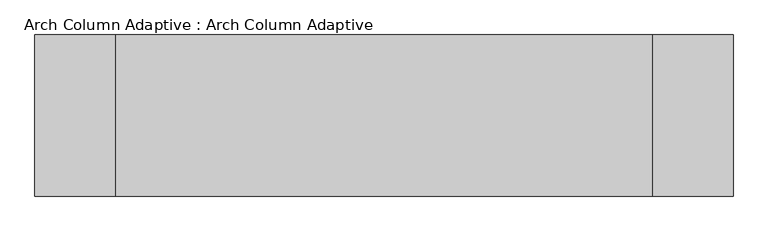
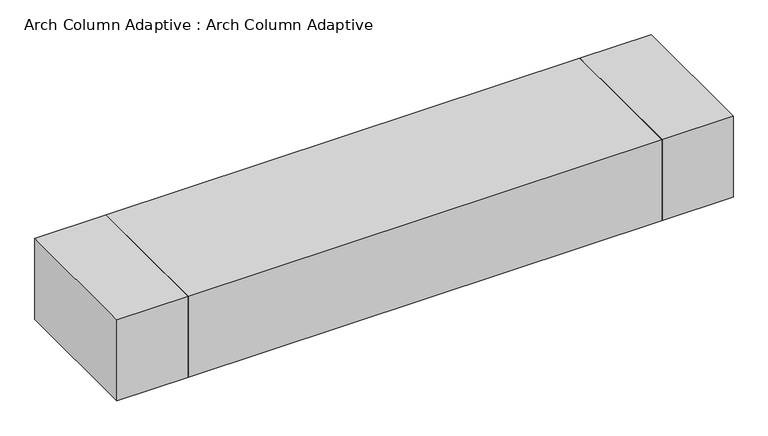
"""IFC4 building model written with IfcOpenShell, lengths in millimetres: proxy geometry, Arch Column Adaptive : Arch Column Adaptive."""

from ifc_helpers import new_model, si_unit, frame, origin, place, context, project, spatial, polyline, outline, extrude, source, transform, mapped, element, save


def arch_column_adaptive_arch_column_adaptive_9be84d25(model_context):
    return source(origin(), model_context, "Body", "SweptSolid", [
        extrude(outline(polyline([(5000.0, -1500.0), (5000.0, 1500.0), (6500.0, 1500.0), (6500.0, -1500.0), (5000.0, -1500.0)])), frame((0.0, 0.0, 79290.0), z_axis=(0.0, 0.0, 1.0), x_axis=(1.0, 0.0, 0.0)), (0.0, 0.0, 1.0), 1800.0),
        extrude(outline(polyline([(-5000.0, 1500.0), (-5000.0, -1500.0), (-6500.0, -1500.0), (-6500.0, 1500.0), (-5000.0, 1500.0)])), frame((0.0, 0.0, 79290.0), z_axis=(0.0, 0.0, 1.0), x_axis=(1.0, 0.0, 0.0)), (0.0, 0.0, 1.0), 1800.0),
        extrude(outline(polyline([(-5000.0, -1500.0), (-5000.0, 1500.0), (5000.0, 1500.0), (5000.0, -1500.0), (-5000.0, -1500.0)])), frame((0.0, 0.0, 79290.0), z_axis=(0.0, 0.0, 1.0), x_axis=(1.0, 0.0, 0.0)), (0.0, 0.0, 1.0), 1800.0),
    ])


if __name__ == "__main__":
    model = new_model("IFC4")
    model_context = context("Model", 3, world=origin())
    ifc_project = project(units=[si_unit("LENGTHUNIT", "METRE", prefix="MILLI")], contexts=[model_context])
    site = spatial("IfcSite", under=ifc_project)
    building = spatial("IfcBuilding", under=site)
    placement = place(None, origin())
    arch_column_adaptive_arch_column_adaptive_shape = arch_column_adaptive_arch_column_adaptive_9be84d25(model_context)
    element("IfcBuildingElementProxy", 1, Name="Arch Column Adaptive : Arch Column Adaptive", ObjectType="Arch Column Adaptive : Arch Column Adaptive", at=placement, inside=building, context=model_context, shape_type="MappedRepresentation", body=[
        mapped(arch_column_adaptive_arch_column_adaptive_shape, transform((0.0, 0.0, 0.0), x_axis=(1.0, 0.0, 0.0), y_axis=(0.0, 1.0, 0.0), z_axis=(0.0, 0.0, 1.0))),
    ])
    save(model, "model.ifc")

# Revit data of these elements
# Type "Arch Column Adaptive : Arch Column Adaptive"
#   Top Width = 3000 mm
#   Length [instance default] = 21000 mm
#   Height [instance default] = 50000 mm
#   Default Elevation = 0
# Element 1 (IfcBuildingElementProxy, "Arch Column Adaptive : Arch Column Adaptive")
#   Height = 79290 mm
